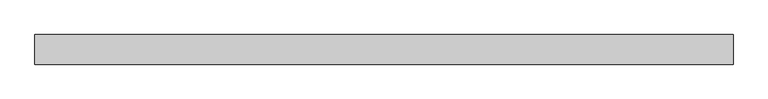
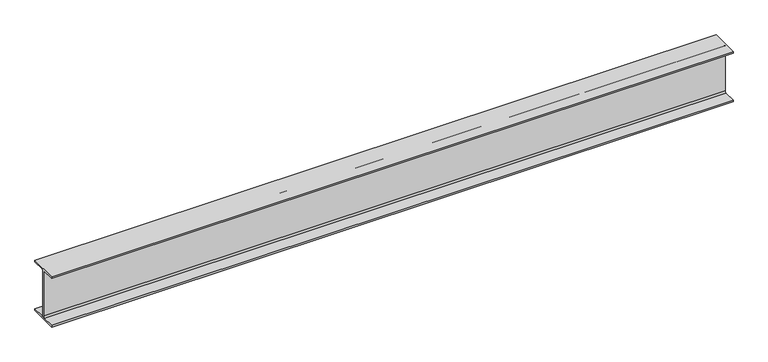
"""IFC4 building model written with IfcOpenShell, lengths in millimetres: beam geometry, Old_Steel Beam_H-KSD3502 : H_SB_ASB_H-200×200x8x12."""

from ifc_helpers import new_model, si_unit, point, frame, frame_2d, origin, place, context, project, spatial, polyline, circle_curve, trimmed, segment, composite_curve, outline, extrude, source, transform, mapped, element, save


def beam_e3e9dac9(model_context):
    return source(origin(), model_context, "Body", "SweptSolid", [
        extrude(outline(composite_curve([segment(polyline([(82.5, -141.5), (82.5, -151.7), (-82.5, -151.7), (-82.5, -141.5), (-11.9, -141.5)]), True, "CONTINUOUS"), segment(trimmed(circle_curve(frame_2d((-11.9, -132.6)), 8.9), [point((-11.9, -141.5))], [point((-3.0, -132.6))], True, "CARTESIAN"), True, "CONTINUOUS"), segment(polyline([(-3.0, -132.6), (-3.0, 132.6)]), True, "CONTINUOUS"), segment(trimmed(circle_curve(frame_2d((-11.9, 132.6)), 8.9), [point((-3.0, 132.6))], [point((-11.9, 141.5))], True, "CARTESIAN"), True, "CONTINUOUS"), segment(polyline([(-11.9, 141.5), (-82.5, 141.5), (-82.5, 151.7), (82.5, 151.7), (82.5, 141.5), (11.9, 141.5)]), True, "CONTINUOUS"), segment(trimmed(circle_curve(frame_2d((11.9, 132.6)), 8.9), [point((11.9, 141.5))], [point((3.0, 132.6))], True, "CARTESIAN"), True, "CONTINUOUS"), segment(polyline([(3.0, 132.6), (3.0, -132.6)]), True, "CONTINUOUS"), segment(trimmed(circle_curve(frame_2d((11.9, -132.6)), 8.9), [point((3.0, -132.6))], [point((11.9, -141.5))], True, "CARTESIAN"), True, "CONTINUOUS"), segment(polyline([(11.9, -141.5), (82.5, -141.5)]), True, "CONTINUOUS")], self_intersect=False)), frame((-1898.8220866, 0.0, 0.0), z_axis=(1.0, 0.0, 0.0), x_axis=(0.0, 1.0, 0.0)), (0.0, 0.0, 1.0), 3882.4854417),
    ])


if __name__ == "__main__":
    model = new_model("IFC4")
    model_context = context("Model", 3, world=origin())
    ifc_project = project(units=[si_unit("LENGTHUNIT", "METRE", prefix="MILLI")], contexts=[model_context])
    site = spatial("IfcSite", under=ifc_project)
    building = spatial("IfcBuilding", under=site)
    placement = place(None, origin())
    beam_shape = beam_e3e9dac9(model_context)
    element("IfcBeam", 1, ObjectType="Old_Steel Beam_H-KSD3502 : H_SB_ASB_H-200×200x8x12", at=placement, inside=building, context=model_context, shape_type="MappedRepresentation", body=[
        mapped(beam_shape, transform((0.0, 0.0, 0.0), x_axis=(1.0, 0.0, 0.0), y_axis=(0.0, 1.0, 0.0), z_axis=(0.0, 0.0, 1.0))),
    ])
    save(model, "model.ifc")

# Revit data of these elements
# Type "Old_Steel Beam_H-KSD3502 : H_SB_ASB_H-200×200x8x12"
#   Width = 20.0 cm
#   Web Thickness = 0.8 cm
#   Web Fillet = 1.3 cm
#   Warping Constant = 141376.0 cm⁶
#   Torsional Moment of Inertia = 26.2485 cm⁴
#   Torsional Modulus = 1.0 cm³
#   Section Area = 63.53 cm²
#   Plastic Modulus weak axis = 244.0 cm³
#   Plastic Modulus strong axis = 525.0 cm³
#   Perimeter = 1.16 m²/m
#   Nominal Weight = 49.90 kgf/m
#   Moment of Inertia weak axis = 1600.00 cm⁴
#   Moment of Inertia strong axis = 4720.00 cm⁴
#   Height = 20.0 cm
#   Flange Thickness = 1.2 cm
#   Elastic Modulus weak axis = 160.0 cm³
#   Elastic Modulus strong axis = 472.0 cm³
#   Centroid Vertical = 10.0 cm
#   Centroid Horizontal = 10.0 cm
#   Length [instance default] = 1.5240 m
#   Structural Material [instance default] = Steel, 45-345
#   Assembly Code = ""
# Element 1 (IfcBeam, "Old_Steel Beam_H-KSD3502 : H_SB_ASB_H-200×200x8x12")
#   Structural Material = none
# Materials
#   "Steel, 45-345": class "Metal", colour RGB 189 187 185, transparency 0, Description = "Steel 345 MPa", Cost = 0
